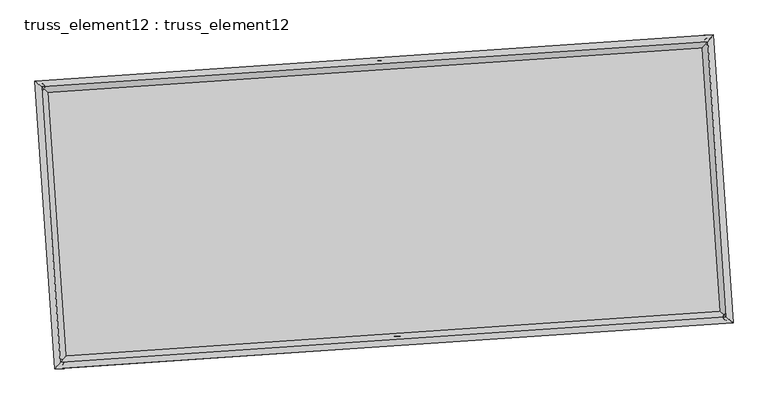
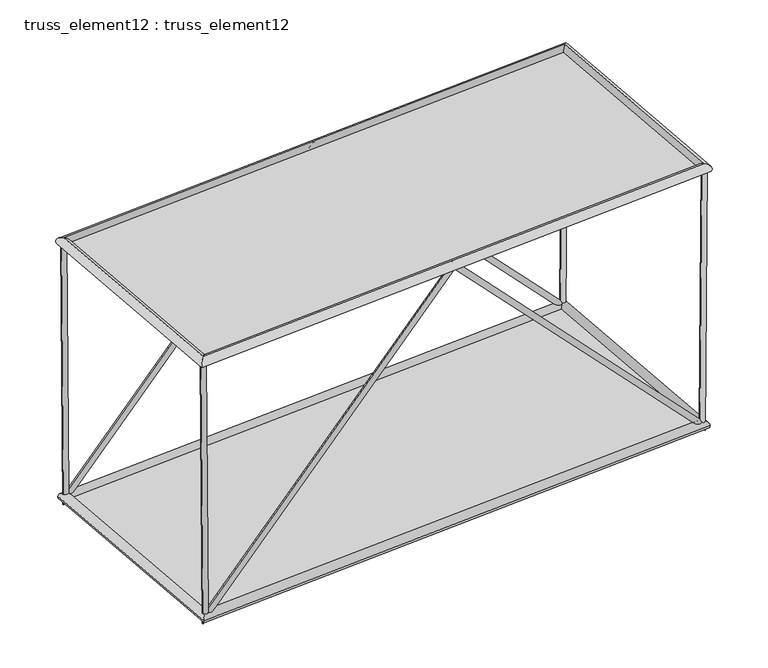
"""IFC4 building model written with IfcOpenShell, lengths in millimetres: plate geometry, truss_element12 : truss_element12."""

from ifc_helpers import new_model, si_unit, frame, origin, origin_with_axes, place, context, project, spatial, polyline, circle_curve, ellipse_curve, outline, extrude, source, transform, mapped, element, save
from ifc_brep_helpers import plane_surface, cylinder_surface, advanced_brep


def truss_element12_truss_element12_d45aceee(model_context):
    return source(origin(), model_context, "Body", "SolidModel", [
        advanced_brep(
        [(-3703.928569, 2273.5656051, 5000.2372149), (-3803.0288933, 2260.2045576, 4999.4573966), (-3665.9008305, 2276.158572, 123.1954643), (-3763.0860523, 2262.9281081, -123.1954643), (1064.0423078, 2598.6754144, 5071.9675631), (1064.4856887, 2592.1018738, 4927.7219862), (5793.3553828, 2921.1492952, 123.190924), (5891.4055943, 2921.2311933, -123.190924), (5832.0084136, 2923.7848984, 5000.2385631), (5932.0050418, 2923.9995153, 4999.445924)],
        [
            (0, 1, circle_curve(frame((-3753.4787312, 2266.8850813, 4999.8473058), z_axis=(-0.007797057947619092, -0.0005316517420559234, 0.9999694611505827), x_axis=(-0.13361054039340575, 0.9910337826601868, -0.0005149000133264984)), 50.0)),
            (1, 0, circle_curve(frame((-3753.4787312, 2266.8850813, 4999.8473058), z_axis=(-0.007797057947619092, -0.0005316517420559234, 0.9999694611505827), x_axis=(-0.13361054039340575, 0.9910337826601868, -0.0005149000133264984)), 50.0)),
            (0, 2),
            (2, 3, ellipse_curve(frame((-3714.4934414, 2269.54334, 0.0), z_axis=(-0.9272265170481931, -0.06322405147954359, 0.36912559569500086), x_axis=(0.3682704778911504, 0.02511096396025113, 0.9293795212951547)), 132.8453216, 50.0)),
            (3, 1),
            (3, 2, ellipse_curve(frame((-3714.4934414, 2269.54334, 0.0), z_axis=(-0.9272265170481931, -0.06322405147954359, 0.36912559569500086), x_axis=(0.3682704778911504, 0.02511096396025113, 0.9293795212951547)), 132.8453216, 50.0)),
            (2, 4),
            (4, 5, ellipse_curve(frame((1064.2639983, 2595.3886441, 4999.8447747), z_axis=(-0.9976833955149683, -0.06802823819052367, 3.350248636381204e-05), x_axis=(-3.342487437246443e-05, -2.2791151238907973e-06, -0.9999999994387918)), 72.2798352, 50.0)),
            (5, 3),
            (5, 4, ellipse_curve(frame((1064.2639983, 2595.3886441, 4999.8447747), z_axis=(-0.9976833955149683, -0.06802823819052367, 3.350248636381204e-05), x_axis=(-3.342487437246443e-05, -2.2791151238907973e-06, -0.9999999994387918)), 72.2798352, 50.0)),
            (4, 6),
            (6, 7, ellipse_curve(frame((5842.3804885, 2921.1902443, 0.0), z_axis=(-0.9272625104149095, -0.06322650573039636, -0.3690347487055439), x_axis=(-0.36817984135818577, -0.02510478379960957, 0.9294155982378584)), 132.8352693, 50.0)),
            (7, 5),
            (7, 6, ellipse_curve(frame((5842.3804885, 2921.1902443, 0.0), z_axis=(-0.9272625104149095, -0.06322650573039636, -0.3690347487055439), x_axis=(-0.36817984135818577, -0.02510478379960957, 0.9294155982378584)), 132.8352693, 50.0)),
            (8, 9, circle_curve(frame((5882.0067277, 2923.8922069, 4999.8422436), z_axis=(0.007925247840658631, 0.0005403925235672647, 0.9999684487135505), x_axis=(-0.0021503844868466107, 0.9999975509646185, -0.0005233653829670034)), 50.0)),
            (9, 8, circle_curve(frame((5882.0067277, 2923.8922069, 4999.8422436), z_axis=(0.007925247840658631, 0.0005403925235672647, 0.9999684487135505), x_axis=(-0.0021503844868466107, 0.9999975509646185, -0.0005233653829670034)), 50.0)),
            (6, 8),
            (9, 7),
        ],
        [
            plane_surface(frame((-3753.4787312, 2316.8850743, 4999.8738891), z_axis=(-0.007797057947618262, -0.0005316517420571678, 0.9999694611505827), x_axis=(0.9999696024816762, -4.14544545179751e-06, 0.0077970568456180375))),
            cylinder_surface(frame((-3753.4787312, 2266.8850813, 4999.8473058), z_axis=(-0.007797057947619092, -0.0005316517420559234, 0.9999694611505827), x_axis=(-0.13361054039340575, 0.9910337826601868, -0.0005149000133264984)), 50.0),
            cylinder_surface(frame((-3714.4934414, 2269.54334, 0.0), z_axis=(-0.6901774781348229, -0.04706057862379895, -0.7221082679315127), x_axis=(-0.020414722847387493, 0.9987521751610632, -0.04557775446541166)), 50.0),
            cylinder_surface(frame((1064.2639983, 2595.3886441, 4999.8447747), z_axis=(-0.690129203829239, -0.0470572869824086, 0.7221546190144297), x_axis=(-0.11534918223811355, 0.992278955254875, -0.04557456653981777)), 50.0),
            plane_surface(frame((5882.0067277, 2873.8922142, 4999.869264), z_axis=(0.007925247840657143, 0.0005403925235714975, 0.9999684487135506), x_axis=(0.9999685947301866, -4.282879185524275e-06, -0.007925246683402767))),
            cylinder_surface(frame((5842.3804885, 2921.1902443, 0.0), z_axis=(-0.007925247840658633, -0.0005403925235672648, -0.9999684487135507), x_axis=(-0.0021503844868466107, 0.9999975509646185, -0.0005233653829670034)), 50.0),
        ],
        [
            (0, [[1, 2]]),
            (1, [[-1, 3, 4, 5]]),
            (1, [[-2, -5, 6, -3]]),
            (2, [[-4, 7, 8, 9]]),
            (2, [[-6, -9, 10, -7]]),
            (3, [[-8, 11, 12, 13]]),
            (3, [[-10, -13, 14, -11]]),
            (4, [[15, 16]]),
            (5, [[-12, 17, -16, 18]]),
            (5, [[-14, -18, -15, -17]]),
        ],
    ),
        advanced_brep(
        [(-3431.815616, -1717.1679792, 5000.2372149), (-3530.9159404, -1730.5290267, 4999.4573966), (-3393.7878776, -1714.5750123, 123.1954643), (-3490.9730994, -1727.8054762, -123.1954643), (1336.1552607, -1392.0581699, 5071.9675631), (1336.5986417, -1398.6317105, 4927.7219862), (6065.4683357, -1069.5842891, 123.190924), (6163.5185472, -1069.502391, -123.190924), (6104.1213665, -1066.9486859, 5000.2385631), (6204.1179947, -1066.734069, 4999.445924)],
        [
            (0, 1, circle_curve(frame((-3481.3657782, -1723.848503, 4999.8473058), z_axis=(-0.00779705794761937, -0.0005316517420559672, 0.9999694611505827), x_axis=(-0.13361054039340567, 0.9910337826601868, -0.0005149000133264915)), 50.0)),
            (1, 0, circle_curve(frame((-3481.3657782, -1723.848503, 4999.8473058), z_axis=(-0.00779705794761937, -0.0005316517420559672, 0.9999694611505827), x_axis=(-0.13361054039340567, 0.9910337826601868, -0.0005149000133264915)), 50.0)),
            (0, 2),
            (2, 3, ellipse_curve(frame((-3442.3804885, -1721.1902443, 0.0), z_axis=(-0.9272265170481933, -0.06322405147954362, 0.3691255956950004), x_axis=(0.36827047789114986, 0.025110963960251077, 0.9293795212951548)), 132.8453216, 50.0)),
            (3, 1),
            (3, 2, ellipse_curve(frame((-3442.3804885, -1721.1902443, 0.0), z_axis=(-0.9272265170481933, -0.06322405147954362, 0.3691255956950004), x_axis=(0.36827047789114986, 0.025110963960251077, 0.9293795212951548)), 132.8453216, 50.0)),
            (2, 4),
            (4, 5, ellipse_curve(frame((1336.3769512, -1395.3449402, 4999.8447747), z_axis=(-0.9976833955149683, -0.06802823819052392, 3.350248636349106e-05), x_axis=(-3.3424874372156944e-05, -2.2791151236217474e-06, -0.9999999994387918)), 72.2798352, 50.0)),
            (5, 3),
            (5, 4, ellipse_curve(frame((1336.3769512, -1395.3449402, 4999.8447747), z_axis=(-0.9976833955149683, -0.06802823819052392, 3.350248636349106e-05), x_axis=(-3.3424874372156944e-05, -2.2791151236217474e-06, -0.9999999994387918)), 72.2798352, 50.0)),
            (4, 6),
            (6, 7, ellipse_curve(frame((6114.4934414, -1069.54334, 0.0), z_axis=(-0.9272625104149094, -0.06322650573039663, -0.36903474870554415), x_axis=(-0.36817984135818593, -0.025104783799609856, 0.9294155982378581)), 132.8352693, 50.0)),
            (7, 5),
            (7, 6, ellipse_curve(frame((6114.4934414, -1069.54334, 0.0), z_axis=(-0.9272625104149094, -0.06322650573039663, -0.36903474870554415), x_axis=(-0.36817984135818593, -0.025104783799609856, 0.9294155982378581)), 132.8352693, 50.0)),
            (8, 9, circle_curve(frame((6154.1196806, -1066.8413774, 4999.8422436), z_axis=(0.007925247840658525, 0.0005403925235671139, 0.9999684487135506), x_axis=(-0.0021503844868468744, 0.9999975509646185, -0.0005233653829668508)), 50.0)),
            (9, 8, circle_curve(frame((6154.1196806, -1066.8413774, 4999.8422436), z_axis=(0.007925247840658525, 0.0005403925235671139, 0.9999684487135506), x_axis=(-0.0021503844868468744, 0.9999975509646185, -0.0005233653829668508)), 50.0)),
            (6, 8),
            (9, 7),
        ],
        [
            plane_surface(frame((-3481.3657782, -1673.84851, 4999.8738891), z_axis=(-0.007797057947618262, -0.0005316517420571707, 0.9999694611505827), x_axis=(0.9999696024816762, -4.14544545179751e-06, 0.0077970568456180375))),
            cylinder_surface(frame((-3481.3657782, -1723.848503, 4999.8473058), z_axis=(-0.00779705794761937, -0.0005316517420559672, 0.9999694611505827), x_axis=(-0.13361054039340567, 0.9910337826601868, -0.0005149000133264915)), 50.0),
            cylinder_surface(frame((-3442.3804885, -1721.1902443, 0.0), z_axis=(-0.6901774781348227, -0.04706057862379893, -0.7221082679315131), x_axis=(-0.020414722847387486, 0.9987521751610632, -0.04557775446541162)), 50.0),
            cylinder_surface(frame((1336.3769512, -1395.3449402, 4999.8447747), z_axis=(-0.690129203829239, -0.047057286982408957, 0.7221546190144295), x_axis=(-0.11534918223811402, 0.992278955254875, -0.04557456653981774)), 50.0),
            plane_surface(frame((6154.1196806, -1116.8413701, 4999.869264), z_axis=(0.007925247840657143, 0.0005403925235715004, 0.9999684487135506), x_axis=(0.9999685947301866, -4.282879185524275e-06, -0.007925246683402767))),
            cylinder_surface(frame((6114.4934414, -1069.54334, 0.0), z_axis=(-0.007925247840658525, -0.0005403925235671139, -0.9999684487135506), x_axis=(-0.0021503844868468744, 0.9999975509646185, -0.0005233653829668508)), 50.0),
        ],
        [
            (0, [[1, 2]]),
            (1, [[-1, 3, 4, 5]]),
            (1, [[-2, -5, 6, -3]]),
            (2, [[-4, 7, 8, 9]]),
            (2, [[-6, -9, 10, -7]]),
            (3, [[-8, 11, 12, 13]]),
            (3, [[-10, -13, 14, -11]]),
            (4, [[15, 16]]),
            (5, [[-12, 17, -16, 18]]),
            (5, [[-14, -18, -15, -17]]),
        ],
    ),
        advanced_brep(
        [(-3481.3671131, -1723.8499825, 4909.8473058), (-3481.3644433, -1723.8470234, 5089.8473057), (-3753.4772078, 2266.8837967, 5089.8473057), (-3753.4802545, 2266.886366, 4909.8473058), (5882.0054869, 2923.8907338, 5089.8422436), (5882.0079685, 2923.89368, 4909.8422436), (6154.1182514, -1066.8400864, 5089.8422436), (6154.1211099, -1066.8426685, 4909.8422436)],
        [
            (0, 1, ellipse_curve(frame((-3481.3657782, -1723.848503, 4999.8473058), z_axis=(-0.7535719234053597, 0.6573654662780887, 3.7063136846259504e-07), x_axis=(-0.657365466277985, -0.7535719234054503, 3.7063136846263464e-07)), 127.2792206, 90.0)),
            (1, 2),
            (2, 3, ellipse_curve(frame((-3753.4787312, 2266.8850813, 4999.8473058), z_axis=(-0.6573654662779852, -0.7535719234054502, 3.7063136846267133e-07), x_axis=(0.7535719234053597, -0.6573654662780887, -3.706313684626316e-07)), 127.2792206, 90.0)),
            (3, 0),
            (1, 0, ellipse_curve(frame((-3481.3657782, -1723.848503, 4999.8473058), z_axis=(-0.7535719234053597, 0.6573654662780887, 3.7063136846259504e-07), x_axis=(-0.657365466277985, -0.7535719234054503, 3.7063136846263464e-07)), 127.2792206, 90.0)),
            (3, 2, ellipse_curve(frame((-3753.4787312, 2266.8850813, 4999.8473058), z_axis=(-0.6573654662779852, -0.7535719234054502, 3.7063136846267133e-07), x_axis=(0.7535719234053597, -0.6573654662780887, -3.706313684626316e-07)), 127.2792206, 90.0)),
            (2, 4),
            (4, 5, ellipse_curve(frame((5882.0067277, 2923.8922069, 4999.8422436), z_axis=(-0.7535719234053598, 0.6573654662780888, 3.7063136846266847e-07), x_axis=(-0.6573654662779853, -0.7535719234054502, 3.706313684626346e-07)), 127.2792206, 90.0)),
            (5, 3),
            (5, 4, ellipse_curve(frame((5882.0067277, 2923.8922069, 4999.8422436), z_axis=(-0.7535719234053598, 0.6573654662780888, 3.7063136846266847e-07), x_axis=(-0.6573654662779853, -0.7535719234054502, 3.706313684626346e-07)), 127.2792206, 90.0)),
            (4, 6),
            (6, 7, ellipse_curve(frame((6154.1196806, -1066.8413774, 4999.8422436), z_axis=(0.6573654662779854, 0.75357192340545, -3.7063136846259806e-07), x_axis=(-0.7535719234053595, 0.657365466278089, 3.706313684626316e-07)), 127.2792206, 90.0)),
            (7, 5),
            (7, 6, ellipse_curve(frame((6154.1196806, -1066.8413774, 4999.8422436), z_axis=(0.6573654662779854, 0.75357192340545, -3.7063136846259806e-07), x_axis=(-0.7535719234053595, 0.657365466278089, 3.706313684626316e-07)), 127.2792206, 90.0)),
            (6, 1),
            (0, 7),
        ],
        [
            cylinder_surface(frame((-3481.3657782, -1723.848503, 4999.8473058), z_axis=(0.06802823822870004, -0.9976833960748767, 0.0), x_axis=(-0.9976833959485084, -0.06802823822008346, 1.5916136040858972e-05)), 90.0),
            cylinder_surface(frame((-3753.4787312, 2266.8850813, 4999.8473058), z_axis=(-0.9976833960747399, -0.06802823822868953, 5.241519079207817e-07), x_axis=(-0.06802823821259144, 0.9976833959572435, 1.5391984133000304e-05)), 90.0),
            cylinder_surface(frame((5882.0067277, 2923.8922069, 4999.8422436), z_axis=(-0.06802823822869983, 0.9976833960748769, 0.0), x_axis=(0.9976833959646066, 0.06802823822118093, 1.4867832225141635e-05)), 90.0),
            cylinder_surface(frame((6154.1196806, -1066.8413774, 4999.8422436), z_axis=(0.9976833960747399, 0.06802823822868947, -5.241519079207299e-07), x_axis=(0.06802823822868947, -0.9976833959561459, 1.5391984133000304e-05)), 90.0),
        ],
        [
            (0, [[1, 2, 3, 4]]),
            (0, [[5, -4, 6, -2]]),
            (1, [[-3, 7, 8, 9]]),
            (1, [[-6, -9, 10, -7]]),
            (2, [[-8, 11, 12, 13]]),
            (2, [[-10, -13, 14, -11]]),
            (3, [[-12, 15, -1, 16]]),
            (3, [[-14, -16, -5, -15]]),
        ],
    ),
        advanced_brep(
        [(-3358.7115243, -1625.2761972, 0.0), (-3526.0494527, -1817.1042913, 0.0), (-3810.4074885, 2353.2123043, 0.0), (-3618.5793943, 2185.8743758, 0.0), (5926.0494527, 3017.1042913, 0.0), (5758.7115243, 2825.2761972, 0.0), (6210.4074885, -1153.2123043, 0.0), (6018.5793943, -985.8743758, 0.0)],
        [
            (0, 1, ellipse_curve(frame((-3442.3804885, -1721.1902443, 0.0), z_axis=(-0.7535719234054588, 0.6573654662780799, 0.0), x_axis=(-0.6573654662780798, -0.7535719234054586, 0.0)), 127.2792206, 90.0)),
            (1, 2),
            (2, 3, ellipse_curve(frame((-3714.4934414, 2269.54334, 0.0), z_axis=(-0.6573654662780802, -0.7535719234054585, 0.0), x_axis=(0.7535719234054586, -0.6573654662780801, 0.0)), 127.2792206, 90.0)),
            (3, 0),
            (1, 0, ellipse_curve(frame((-3442.3804885, -1721.1902443, 0.0), z_axis=(-0.7535719234054588, 0.6573654662780799, 0.0), x_axis=(-0.6573654662780798, -0.7535719234054586, 0.0)), 127.2792206, 90.0)),
            (3, 2, ellipse_curve(frame((-3714.4934414, 2269.54334, 0.0), z_axis=(-0.6573654662780802, -0.7535719234054585, 0.0), x_axis=(0.7535719234054586, -0.6573654662780801, 0.0)), 127.2792206, 90.0)),
            (2, 4),
            (4, 5, ellipse_curve(frame((5842.3804885, 2921.1902443, 0.0), z_axis=(-0.7535719234054586, 0.6573654662780799, 0.0), x_axis=(-0.6573654662780802, -0.7535719234054585, 0.0)), 127.2792206, 90.0)),
            (5, 3),
            (5, 4, ellipse_curve(frame((5842.3804885, 2921.1902443, 0.0), z_axis=(-0.7535719234054586, 0.6573654662780799, 0.0), x_axis=(-0.6573654662780802, -0.7535719234054585, 0.0)), 127.2792206, 90.0)),
            (4, 6),
            (6, 7, ellipse_curve(frame((6114.4934414, -1069.54334, 0.0), z_axis=(0.6573654662780798, 0.7535719234054586, 0.0), x_axis=(-0.7535719234054585, 0.6573654662780801, 0.0)), 127.2792206, 90.0)),
            (7, 5),
            (7, 6, ellipse_curve(frame((6114.4934414, -1069.54334, 0.0), z_axis=(0.6573654662780798, 0.7535719234054586, 0.0), x_axis=(-0.7535719234054585, 0.6573654662780801, 0.0)), 127.2792206, 90.0)),
            (6, 1),
            (0, 7),
        ],
        [
            cylinder_surface(frame((-3442.3804885, -1721.1902443, 0.0), z_axis=(0.06802823822870296, -0.9976833960748764, 0.0), x_axis=(-0.9976833960748764, -0.06802823822870296, 0.0)), 90.0),
            cylinder_surface(frame((-3714.4934414, 2269.54334, 0.0), z_axis=(-0.9976833960748765, -0.06802823822870162, 0.0), x_axis=(-0.06802823822870162, 0.9976833960748765, 0.0)), 90.0),
            cylinder_surface(frame((5842.3804885, 2921.1902443, 0.0), z_axis=(-0.06802823822870298, 0.9976833960748764, 0.0), x_axis=(0.9976833960748764, 0.06802823822870298, 0.0)), 90.0),
            cylinder_surface(frame((6114.4934414, -1069.54334, 0.0), z_axis=(0.9976833960748765, 0.06802823822870185, 0.0), x_axis=(0.06802823822870185, -0.9976833960748765, 0.0)), 90.0),
        ],
        [
            (0, [[1, 2, 3, 4]]),
            (0, [[5, -4, 6, -2]]),
            (1, [[-3, 7, 8, 9]]),
            (1, [[-6, -9, 10, -7]]),
            (2, [[-8, 11, 12, 13]]),
            (2, [[-10, -13, 14, -11]]),
            (3, [[-12, 15, -1, 16]]),
            (3, [[-14, -16, -5, -15]]),
        ],
    ),
        extrude(outline(polyline([(-3442.3804885, -1721.1902443), (-3714.4934414, 2269.54334), (5842.3804885, 2921.1902443), (6114.4934414, -1069.54334), (-3442.3804885, -1721.1902443)])), origin_with_axes(), (0.0, 0.0, 1.0), 20.0),
        extrude(outline(polyline([(-2000.0000001, 4828.9294463), (1999.9999999, 4828.9294464), (2000.0, -4828.9294464), (-2000.0, -4828.9294464), (-2000.0000001, 4828.9294463)])), frame((1200.3204747, 600.021852, 4999.8447747), z_axis=(5.229376555535051e-07, 3.56571308600623e-08, 0.9999999999998627), x_axis=(-0.06802823822870292, 0.9976833960748765, 0.0)), (0.0, 0.0, 1.0), 20.0),
    ])


if __name__ == "__main__":
    model = new_model("IFC4")
    model_context = context("Model", 3, world=origin())
    ifc_project = project(units=[si_unit("LENGTHUNIT", "METRE", prefix="MILLI")], contexts=[model_context])
    site = spatial("IfcSite", under=ifc_project)
    building = spatial("IfcBuilding", under=site)
    placement = place(None, origin())
    truss_element12_truss_element12_shape = truss_element12_truss_element12_d45aceee(model_context)
    element("IfcPlate", 1, ObjectType="truss_element12 : truss_element12", at=placement, inside=building, context=model_context, shape_type="MappedRepresentation", body=[
        mapped(truss_element12_truss_element12_shape, transform((0.0, 0.0, 0.0), x_axis=(1.0, 0.0, 0.0), y_axis=(0.0, 1.0, 0.0), z_axis=(0.0, 0.0, 1.0))),
    ])
    save(model, "model.ifc")

# Revit data of these elements
# Type "truss_element12 : truss_element12"
#   steellbar1 = 90 mm
#   steelbar2 = 50 mm
#   offset1 = 5000 mm
#   M = Default Roof
# Element 1 (IfcPlate, "truss_element12 : truss_element12")
#   Materials on its faces: "Default Roof"
# Materials
#   "Default Roof": class "Miscellaneous", colour RGB 0 127 0, transparency 0, Comments = "Rendering appearance not upgraded Rendering appearance not upgraded ", Cost = 0
